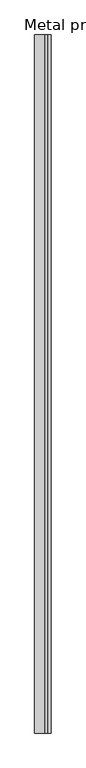
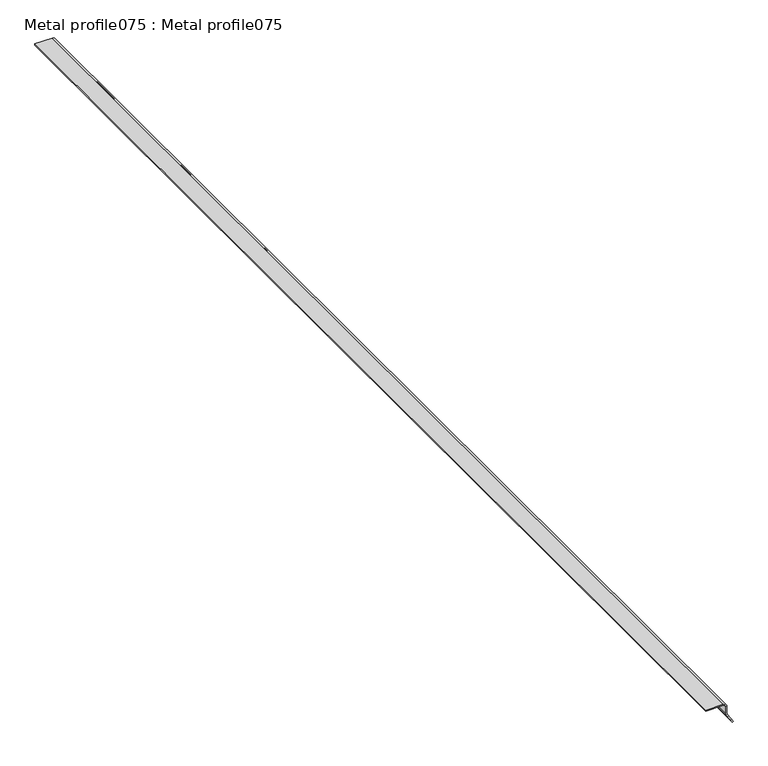
"""IFC4 building model written with IfcOpenShell, lengths in millimetres: proxy geometry, Metal profile075 : Metal profile075."""

from ifc_helpers import new_model, si_unit, point, frame, frame_2d, origin, place, context, project, spatial, polyline, circle_curve, trimmed, segment, composite_curve, outline, extrude, source, transform, mapped, element, save


def metal_profile075_metal_profile075_58743c9b(model_context):
    return source(origin(), model_context, "Body", "SweptSolid", [
        extrude(outline(composite_curve([segment(polyline([(40166.609375, -9813.1152344), (40166.609375, -9783.3685547)]), True, "CONTINUOUS"), segment(trimmed(circle_curve(frame_2d((40162.259375, -9783.3685547)), 4.35), [point((40166.609375, -9783.3685547))], [point((40162.259375, -9779.0185547))], True, "CARTESIAN"), True, "CONTINUOUS"), segment(polyline([(40162.259375, -9779.0185547), (40151.208717, -9779.0185547)]), True, "CONTINUOUS"), segment(trimmed(circle_curve(frame_2d((40151.208717, -9770.6685547)), 8.35), [point((40151.208717, -9779.0185547))], [point((40146.8542568, -9777.7932425))], False, "CARTESIAN"), True, "CONTINUOUS"), segment(polyline([(40146.8542568, -9777.7932425), (40130.8202968, -9767.9936214), (40131.8632813, -9766.2871094), (40147.8972413, -9776.0867304)]), True, "CONTINUOUS"), segment(trimmed(circle_curve(frame_2d((40151.208717, -9770.6685547)), 6.35), [point((40147.8972413, -9776.0867304))], [point((40151.208717, -9777.0185547))], True, "CARTESIAN"), True, "CONTINUOUS"), segment(polyline([(40151.208717, -9777.0185547), (40162.259375, -9777.0185547)]), True, "CONTINUOUS"), segment(trimmed(circle_curve(frame_2d((40162.259375, -9783.3685547)), 6.35), [point((40162.259375, -9777.0185547))], [point((40168.609375, -9783.3685547))], False, "CARTESIAN"), True, "CONTINUOUS"), segment(polyline([(40168.609375, -9783.3685547), (40168.609375, -9813.1152344), (40166.609375, -9813.1152344)]), True, "CONTINUOUS")], self_intersect=False)), frame((0.0, 7982.1531721, 0.0), z_axis=(0.0, 1.0, 0.0), x_axis=(0.0, 0.0, 1.0)), (0.0, 0.0, 1.0), 2000.0),
    ])


if __name__ == "__main__":
    model = new_model("IFC4")
    model_context = context("Model", 3, world=origin())
    ifc_project = project(units=[si_unit("LENGTHUNIT", "METRE", prefix="MILLI")], contexts=[model_context])
    site = spatial("IfcSite", under=ifc_project)
    building = spatial("IfcBuilding", under=site)
    placement = place(None, origin())
    metal_profile075_metal_profile075_shape = metal_profile075_metal_profile075_58743c9b(model_context)
    element("IfcBuildingElementProxy", 1, Name="Metal profile075 : Metal profile075", ObjectType="Metal profile075 : Metal profile075", at=placement, inside=building, context=model_context, shape_type="MappedRepresentation", body=[
        mapped(metal_profile075_metal_profile075_shape, transform((0.0, 0.0, 0.0), x_axis=(1.0, 0.0, 0.0), y_axis=(0.0, 1.0, 0.0), z_axis=(0.0, 0.0, 1.0))),
    ])
    save(model, "model.ifc")

# Revit data of these elements
# Type "Metal profile075 : Metal profile075"
#   NameOverride = "Metal profile075"
# Element 1 (IfcBuildingElementProxy, "Metal profile075 : Metal profile075")
#   Materials on its faces: "ANGLE TRIM"
# Materials
#   "ANGLE TRIM": class "Unassigned", colour RGB 250 255 0, transparency 0
